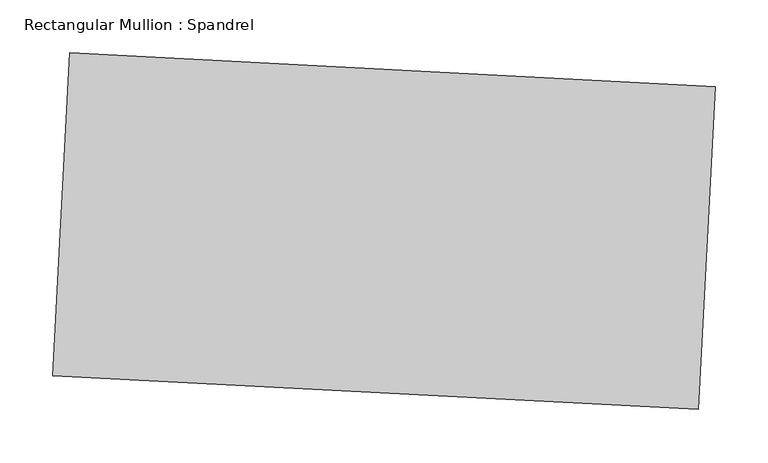
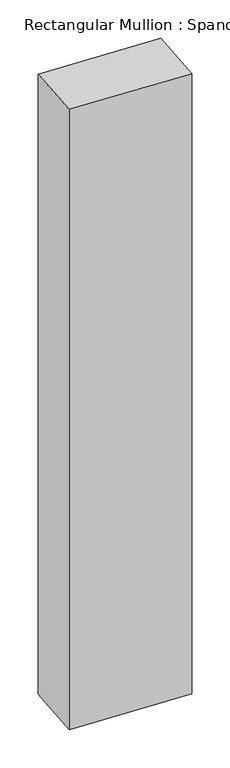
"""IFC4 building model written with IfcOpenShell, lengths in millimetres: member geometry, Rectangular Mullion : Spandrel."""

import ifcopenshell
import ifcopenshell.guid

model = None  # the IFC model being written
_history = None  # IfcOwnerHistory: only IFC2X3 demands one
_inside = {}  # id of a spatial element -> (the spatial element, [elements in it])
_under = {}  # id of a project, library or spatial element -> (it, [spatial elements below it])
_declared = {}  # id of a project -> (the project, [libraries it declares])
_typed = {}  # id of a type object -> (the type object, [elements of that type])
_made_of = {}  # id of a material, layer set ... -> (it, [elements and type objects made of it])


def new_model(schema):
    """Start an empty IFC model of exactly this schema.

    Asked for "IFC4X3", IfcOpenShell would pick the latest addendum, in which some entities
    have other attributes; the version numbers below select the first issue.
    IFC2X3 requires an IfcOwnerHistory on every rooted entity: one is made here for all.
    """
    global model, _history
    if schema == "IFC4X3":
        model = ifcopenshell.file(schema_version=(4, 3, 0, 0))
    else:
        model = ifcopenshell.file(schema=schema)
    _inside.clear()
    _under.clear()
    _declared.clear()
    _typed.clear()
    _made_of.clear()
    _history = None
    if model.schema == "IFC2X3":
        org = make("IfcOrganization", Name="unknown")
        user = make(
            "IfcPersonAndOrganization",
            ThePerson=make("IfcPerson", FamilyName="unknown"),
            TheOrganization=org,
        )
        app = make(
            "IfcApplication",
            ApplicationDeveloper=org,
            Version="unknown",
            ApplicationFullName="unknown",
            ApplicationIdentifier="unknown",
        )
        _history = make(
            "IfcOwnerHistory",
            OwningUser=user,
            OwningApplication=app,
            ChangeAction="ADDED",
            CreationDate=0,
        )
    return model


def make(cls, **values):
    """One entity of the class cls with the attributes given. An attribute that is None is left unset."""
    return model.create_entity(
        cls, **{name: value for name, value in values.items() if value is not None}
    )


def rooted(cls, **values):
    """An entity with a GlobalId (a new one), such as an element, a storey or a relation."""
    return make(cls, GlobalId=ifcopenshell.guid.new(), OwnerHistory=_history, **values)


def si_unit(unit_type, name, prefix=None):
    """IfcSIUnit, for example si_unit("LENGTHUNIT", "METRE", prefix="MILLI")."""
    return make("IfcSIUnit", UnitType=unit_type, Prefix=prefix, Name=name)


def assignment(units):
    """IfcUnitAssignment: the units of a project."""
    return None if units is None else make("IfcUnitAssignment", Units=units)


def point(xyz):
    """IfcCartesianPoint."""
    return None if xyz is None else make("IfcCartesianPoint", Coordinates=xyz)


def direction(xyz):
    """IfcDirection."""
    return None if xyz is None else make("IfcDirection", DirectionRatios=xyz)


def frame(location, z_axis=None, x_axis=None):
    """IfcAxis2Placement3D, a coordinate frame: its origin and axes. An axis left out is left unset."""
    return make(
        "IfcAxis2Placement3D",
        Location=point(location),
        Axis=direction(z_axis),
        RefDirection=direction(x_axis),
    )


def origin():
    """The frame at (0, 0, 0) with its axes left unset."""
    return frame((0.0, 0.0, 0.0))


def place(relative_to, where):
    """IfcLocalPlacement: puts the frame where relative to a parent placement (None: the world)."""
    return make(
        "IfcLocalPlacement", PlacementRelTo=relative_to, RelativePlacement=where
    )


def context(
    kind, dimensions, precision=None, world=None, true_north=None, identifier=None
):
    """IfcGeometricRepresentationContext, for example the 3D "Model" context."""
    return make(
        "IfcGeometricRepresentationContext",
        ContextIdentifier=identifier,
        ContextType=kind,
        CoordinateSpaceDimension=dimensions,
        Precision=precision,
        WorldCoordinateSystem=world,
        TrueNorth=true_north,
    )


def project(units=None, contexts=None):
    """IfcProject with its units and contexts."""
    return rooted(
        "IfcProject",
        Name="project",
        RepresentationContexts=contexts,
        UnitsInContext=assignment(units),
    )


def spatial(cls, under=None, at=None, **own):
    """A site, building, storey or space (cls), placed at a placement, below another one or the project."""
    s = rooted(cls, ObjectPlacement=at, **own)
    if under is not None:
        _under.setdefault(under.id(), (under, []))[1].append(s)
    return s


def polyline(points):
    """IfcPolyline through the points."""
    return make("IfcPolyline", Points=[point(p) for p in points])


def outline(outer, holes=None, kind="AREA"):
    """IfcArbitraryClosedProfileDef: a profile drawn as a closed curve; with holes, ...WithVoids."""
    if holes is None:
        return make("IfcArbitraryClosedProfileDef", ProfileType=kind, OuterCurve=outer)
    return make(
        "IfcArbitraryProfileDefWithVoids",
        ProfileType=kind,
        OuterCurve=outer,
        InnerCurves=holes,
    )


def extrude(swept, where, along, depth):
    """IfcExtrudedAreaSolid: the profile swept, set in the frame where, extruded along a direction by depth."""
    return make(
        "IfcExtrudedAreaSolid",
        SweptArea=swept,
        Position=where,
        ExtrudedDirection=direction(along),
        Depth=depth,
    )


def shape(context_of_items, identifier, shape_type, items):
    """IfcShapeRepresentation: the items that make up one representation, for example the "Body"."""
    return make(
        "IfcShapeRepresentation",
        ContextOfItems=context_of_items,
        RepresentationIdentifier=identifier,
        RepresentationType=shape_type,
        Items=items,
    )


def source(mapping_origin, context_of_items, identifier, shape_type, items):
    """IfcRepresentationMap: a shape defined once, which mapped items show again and again."""
    return make(
        "IfcRepresentationMap",
        MappingOrigin=mapping_origin,
        MappedRepresentation=shape(context_of_items, identifier, shape_type, items),
    )


def transform(
    local_origin,
    x_axis=None,
    y_axis=None,
    z_axis=None,
    scale=None,
    scale2=None,
    scale3=None,
    uniform=True,
):
    """IfcCartesianTransformationOperator3D, or its non-uniform kind. x_axis, y_axis, z_axis: its Axis1, 2, 3."""
    if uniform:
        return make(
            "IfcCartesianTransformationOperator3D",
            Axis1=direction(x_axis),
            Axis2=direction(y_axis),
            LocalOrigin=point(local_origin),
            Scale=scale,
            Axis3=direction(z_axis),
        )
    return make(
        "IfcCartesianTransformationOperator3DnonUniform",
        Axis1=direction(x_axis),
        Axis2=direction(y_axis),
        LocalOrigin=point(local_origin),
        Scale=scale,
        Axis3=direction(z_axis),
        Scale2=scale2,
        Scale3=scale3,
    )


def mapped(mapping_source, mapping_target):
    """IfcMappedItem: shows the shape of a source again, moved by a transform."""
    return make(
        "IfcMappedItem", MappingSource=mapping_source, MappingTarget=mapping_target
    )


def made_of(thing, what):
    """Note that an element or type object is made of a material, layer set ...; save() writes the relation."""
    if what is not None:
        _made_of.setdefault(what.id(), (what, []))[1].append(thing)
    return thing


def element(
    cls,
    number,
    at=None,
    inside=None,
    cuts=None,
    type_object=None,
    material=None,
    context=None,
    identifier="Body",
    shape_type=None,
    held_by="IfcProductDefinitionShape",
    body=None,
    shapes=None,
    **own,
):
    """One element of the class cls, such as IfcWall. Its Tag is "e" and its number.

    at: its placement. inside: the storey or other place that contains it. cuts: it is an
    opening in that element (IfcRelVoidsElement). A single representation is given by context,
    identifier, shape_type and body (its items); several are given by shapes. held_by: the class
    of the entity that holds the representations. save() writes the other relations.
    """
    e = rooted(cls, Tag="e%d" % number, ObjectPlacement=at, **own)
    if body is not None:
        shapes = [shape(context, identifier, shape_type, body)]
    if shapes is not None:
        e.Representation = make(held_by, Representations=shapes)
    if inside is not None:
        _inside.setdefault(inside.id(), (inside, []))[1].append(e)
    if cuts is not None:
        rooted(
            "IfcRelVoidsElement", RelatingBuildingElement=cuts, RelatedOpeningElement=e
        )
    if type_object is not None:
        _typed.setdefault(type_object.id(), (type_object, []))[1].append(e)
    return made_of(e, material)


def aggregate(whole, parts):
    """IfcRelAggregates: a whole, such as a stair, and the parts it consists of."""
    return rooted("IfcRelAggregates", RelatingObject=whole, RelatedObjects=parts)


def save(model, path):
    """Write the relations noted so far, then the file.

    IfcRelAggregates (storeys below a building ...), IfcRelContainedInSpatialStructure (elements
    in a storey), IfcRelDefinesByType, IfcRelAssociatesMaterial and IfcRelDeclares: one each for
    every whole, place, type object, material and project.
    """
    for whole, parts in _under.values():
        aggregate(whole, parts)
    for where, things in _inside.values():
        rooted(
            "IfcRelContainedInSpatialStructure",
            RelatedElements=things,
            RelatingStructure=where,
        )
    for kind, things in _typed.values():
        rooted("IfcRelDefinesByType", RelatedObjects=things, RelatingType=kind)
    for what, things in _made_of.values():
        rooted("IfcRelAssociatesMaterial", RelatedObjects=things, RelatingMaterial=what)
    for by, libraries in _declared.values():
        rooted("IfcRelDeclares", RelatingContext=by, RelatedDefinitions=libraries)
    model.write(path)


def rectangular_mullion_spandrel_e4d64f46(model_context):
    return source(origin(), model_context, "Body", "SweptSolid", [
        extrude(outline(polyline([(7.5582819, 136.2391416), (-8.3937175, -168.1431406), (-617.1582819, -136.2391416), (-601.2062825, 168.1431406), (7.5582819, 136.2391416)])), frame((0.0, 0.0, -3352.8), z_axis=(0.0, 0.0, 1.0), x_axis=(1.0, 0.0, 0.0)), (0.0, 0.0, 1.0), 3352.8),
    ])


if __name__ == "__main__":
    model = new_model("IFC4")
    model_context = context("Model", 3, world=origin())
    ifc_project = project(units=[si_unit("LENGTHUNIT", "METRE", prefix="MILLI")], contexts=[model_context])
    site = spatial("IfcSite", under=ifc_project)
    building = spatial("IfcBuilding", under=site)
    placement = place(None, origin())
    rectangular_mullion_spandrel_shape = rectangular_mullion_spandrel_e4d64f46(model_context)
    element("IfcMember", 1, ObjectType="Rectangular Mullion : Spandrel", at=placement, inside=building, context=model_context, shape_type="MappedRepresentation", body=[
        mapped(rectangular_mullion_spandrel_shape, transform((0.0, 0.0, 0.0), x_axis=(1.0, 0.0, 0.0), y_axis=(0.0, 1.0, 0.0), z_axis=(0.0, 0.0, 1.0))),
    ])
    save(model, "model.ifc")

# Revit data of these elements
# Type "Rectangular Mullion : Spandrel"
#   built-in parameter 1007304 = 1 (stored number, unit not read)
#   built-in parameter 1007301 = 1 (stored number, unit not read)
#   built-in parameter 1007300 = 1 (stored number, unit not read)
# Element 1 (IfcMember, "Rectangular Mullion : Spandrel")
#   Materials on its faces: "Aluminum"
# Materials
#   "Aluminum": class "Metal", colour RGB 247 247 247, transparency 0, Description = "Aluminum 6061", Cost = 0
